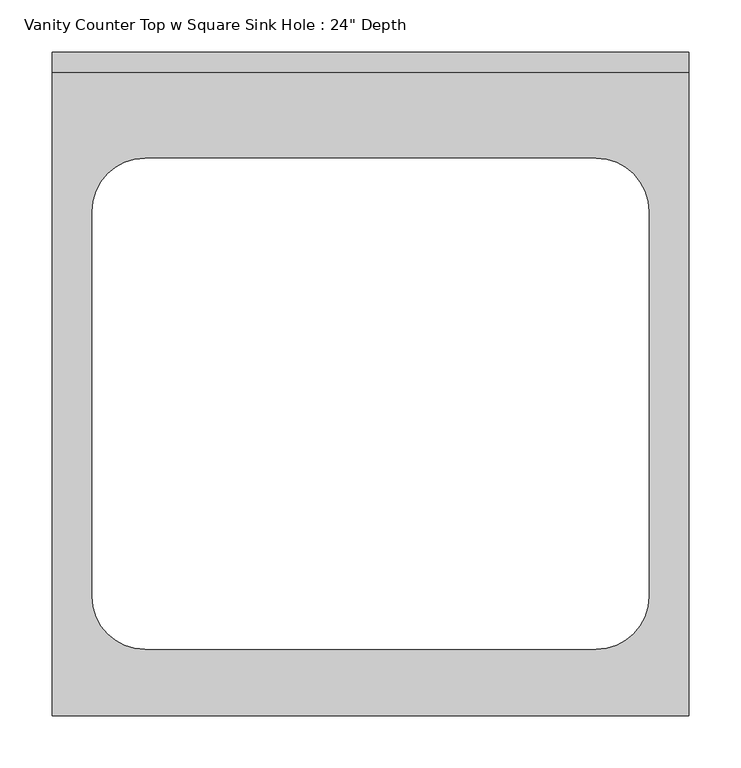
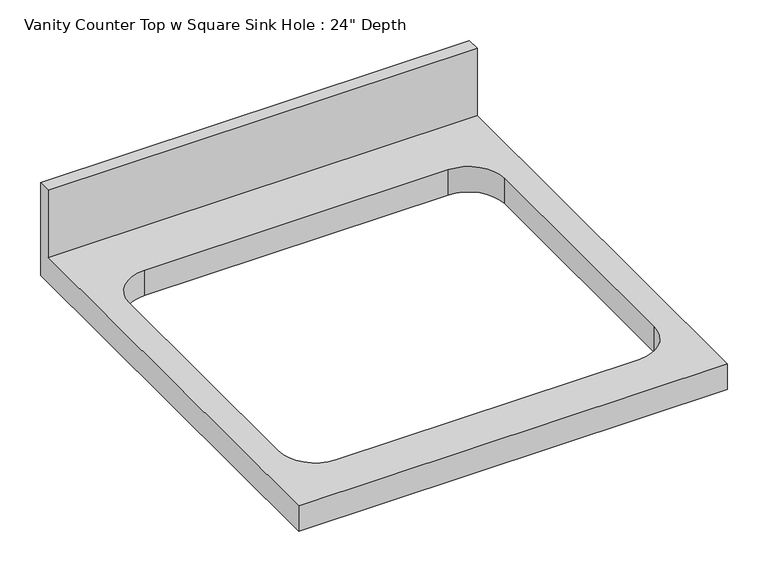
"""IFC4 building model written with IfcOpenShell, lengths in millimetres: furniture geometry."""

from ifc_helpers import new_model, si_unit, frame, origin, place, context, project, spatial, polyline, circle_curve, source, transform, mapped, element, save
from ifc_brep_helpers import plane_surface, revolved_surface, advanced_brep


def furniture_9bca86e0(model_context):
    return source(origin(), model_context, "Body", "AdvancedBrep", [
        advanced_brep(
        [(-1268.7247951, -635.0, 787.4), (-659.1247951, -635.0, 787.4), (-659.1247951, -19.05, 787.4), (-1268.7247951, -19.05, 787.4), (-1230.6247951, -152.4, 787.4), (-1179.8247951, -101.6, 787.4), (-748.0247951, -101.6, 787.4), (-697.2247951, -152.4, 787.4), (-697.2247951, -520.7, 787.4), (-748.0247951, -571.5, 787.4), (-1179.8247951, -571.5, 787.4), (-1230.6247951, -520.7, 787.4), (-659.1247951, 0.0, 749.3), (-659.1247951, -635.0, 749.3), (-1268.7247951, -635.0, 749.3), (-1268.7247951, 0.0, 749.3), (-1179.8247951, -101.6, 749.3), (-1230.6247951, -152.4, 749.3), (-1230.6247951, -520.7, 749.3), (-1179.8247951, -571.5, 749.3), (-748.0247951, -571.5, 749.3), (-697.2247951, -520.7, 749.3), (-697.2247951, -152.4, 749.3), (-748.0247951, -101.6, 749.3), (-1268.7247951, 0.0, 889.0), (-659.1247951, 0.0, 889.0), (-1268.7247951, -19.05, 889.0), (-659.1247951, -19.05, 889.0)],
        [
            (0, 1),
            (1, 2),
            (2, 3),
            (3, 0),
            (4, 5, circle_curve(frame((-1179.8247951, -152.4, 787.4), z_axis=(0.0, 0.0, -1.0), x_axis=(1.0, 0.0, 0.0)), 50.8)),
            (5, 6),
            (6, 7, circle_curve(frame((-748.0247951, -152.4, 787.4), z_axis=(0.0, 0.0, -1.0), x_axis=(1.0, 0.0, 0.0)), 50.8)),
            (7, 8),
            (8, 9, circle_curve(frame((-748.0247951, -520.7, 787.4), z_axis=(0.0, 0.0, -1.0), x_axis=(1.0, 0.0, 0.0)), 50.8)),
            (9, 10),
            (10, 11, circle_curve(frame((-1179.8247951, -520.7, 787.4), z_axis=(0.0, 0.0, -1.0), x_axis=(1.0, 0.0, 0.0)), 50.8)),
            (11, 4),
            (12, 13),
            (13, 14),
            (14, 15),
            (15, 12),
            (16, 17, circle_curve(frame((-1179.8247951, -152.4, 749.3), z_axis=(0.0, 0.0, 1.0), x_axis=(1.0, 0.0, 0.0)), 50.8)),
            (17, 18),
            (18, 19, circle_curve(frame((-1179.8247951, -520.7, 749.3), z_axis=(0.0, 0.0, 1.0), x_axis=(1.0, 0.0, 0.0)), 50.8)),
            (19, 20),
            (20, 21, circle_curve(frame((-748.0247951, -520.7, 749.3), z_axis=(0.0, 0.0, 1.0), x_axis=(1.0, 0.0, 0.0)), 50.8)),
            (21, 22),
            (22, 23, circle_curve(frame((-748.0247951, -152.4, 749.3), z_axis=(0.0, 0.0, 1.0), x_axis=(1.0, 0.0, 0.0)), 50.8)),
            (23, 16),
            (15, 24),
            (24, 25),
            (25, 12),
            (14, 0),
            (3, 26),
            (26, 24),
            (13, 1),
            (25, 27),
            (27, 2),
            (26, 27),
            (4, 17),
            (16, 5),
            (11, 18),
            (10, 19),
            (9, 20),
            (8, 21),
            (7, 22),
            (6, 23),
        ],
        [
            plane_surface(frame((-1268.7247951, 0.0, 787.4), z_axis=(0.0, 0.0, 1.0), x_axis=(-1.0, 0.0, 0.0))),
            plane_surface(frame((-1268.7247951, 0.0, 749.3), z_axis=(0.0, 0.0, -1.0), x_axis=(1.0, 0.0, 0.0))),
            plane_surface(frame((-659.1247951, 0.0, 787.4), z_axis=(0.0, 1.0, 0.0), x_axis=(0.0, 0.0, -1.0))),
            plane_surface(frame((-1268.7247951, 0.0, 787.4), z_axis=(-1.0, 0.0, 0.0), x_axis=(0.0, 0.0, -1.0))),
            plane_surface(frame((-1268.7247951, -635.0, 787.4), z_axis=(0.0, -1.0, 0.0), x_axis=(0.0, 0.0, -1.0))),
            plane_surface(frame((-659.1247951, -635.0, 787.4), z_axis=(1.0, 0.0, 0.0), x_axis=(0.0, 0.0, -1.0))),
            plane_surface(frame((-1268.7247951, 0.0, 889.0), z_axis=(0.0, 0.0, 1.0), x_axis=(0.0, -1.0, 0.0))),
            plane_surface(frame((-1268.7247951, -19.05, 889.0), z_axis=(0.0, -1.0, 0.0), x_axis=(0.0, 0.0, -1.0))),
            revolved_surface(polyline([(-1129.0247951000001, -152.4, 787.4), (-1129.0247951000001, -152.4, 749.3)]), (-1179.8247951, -152.4, 749.3), (0.0, 0.0, 1.0)),
            plane_surface(frame((-1230.6247951, -152.4, 787.4), z_axis=(1.0, 0.0, 0.0), x_axis=(0.0, 0.0, -1.0))),
            revolved_surface(polyline([(-1129.0247951000001, -520.7, 787.4), (-1129.0247951000001, -520.7, 749.3)]), (-1179.8247951, -520.7, 749.3), (0.0, 0.0, 1.0)),
            plane_surface(frame((-1179.8247951, -571.5, 787.4), z_axis=(0.0, 1.0, 0.0), x_axis=(0.0, 0.0, -1.0))),
            revolved_surface(polyline([(-697.2247951, -520.7, 787.4), (-697.2247951, -520.7, 749.3)]), (-748.0247951, -520.7, 749.3), (0.0, 0.0, 1.0)),
            plane_surface(frame((-697.2247951, -520.7, 787.4), z_axis=(-1.0, 0.0, 0.0), x_axis=(0.0, 0.0, -1.0))),
            revolved_surface(polyline([(-697.2247951, -152.4, 787.4), (-697.2247951, -152.4, 749.3)]), (-748.0247951, -152.4, 749.3), (0.0, 0.0, 1.0)),
            plane_surface(frame((-748.0247951, -101.6, 787.4), z_axis=(0.0, -1.0, 0.0), x_axis=(0.0, 0.0, -1.0))),
        ],
        [
            (0, [[1, 2, 3, 4], [5, 6, 7, 8, 9, 10, 11, 12]]),
            (1, [[13, 14, 15, 16], [17, 18, 19, 20, 21, 22, 23, 24]]),
            (2, [[-16, 25, 26, 27]]),
            (3, [[-15, 28, -4, 29, 30, -25]]),
            (4, [[-1, -28, -14, 31]]),
            (5, [[-13, -27, 32, 33, -2, -31]]),
            (6, [[-30, 34, -32, -26]]),
            (7, [[-34, -29, -3, -33]]),
            (8, [[35, -17, 36, -5]]),
            (9, [[-35, -12, 37, -18]]),
            (10, [[-37, -11, 38, -19]]),
            (11, [[-38, -10, 39, -20]]),
            (12, [[-39, -9, 40, -21]]),
            (13, [[-40, -8, 41, -22]]),
            (14, [[-41, -7, 42, -23]]),
            (15, [[-36, -24, -42, -6]]),
        ],
    ),
    ])


if __name__ == "__main__":
    model = new_model("IFC4")
    model_context = context("Model", 3, world=origin())
    ifc_project = project(units=[si_unit("LENGTHUNIT", "METRE", prefix="MILLI")], contexts=[model_context])
    site = spatial("IfcSite", under=ifc_project)
    building = spatial("IfcBuilding", under=site)
    placement = place(None, origin())
    furniture_shape = furniture_9bca86e0(model_context)
    element("IfcFurniture", 1, ObjectType="Vanity Counter Top w Square Sink Hole : 24\" Depth", at=placement, inside=building, context=model_context, shape_type="MappedRepresentation", body=[
        mapped(furniture_shape, transform((0.0, 0.0, 0.0), x_axis=(1.0, 0.0, 0.0), y_axis=(0.0, 1.0, 0.0), z_axis=(0.0, 0.0, 1.0))),
    ])
    save(model, "model.ifc")

# Revit data of these elements
# Type "Vanity Counter Top w Square Sink Hole : 24\" Depth"
#   Assembly Code = "C1030400"
#   Counter Thickness = 0' - 1 1/2"
#   Depth = 2' - 1"
#   Height = 2' - 7"
#   Length [instance default] = 4' - 0"
#   Sink Location [instance default] = 2' - 0"
#   Sink Location To Wall [instance default] = 0' - 4 1/2"
#   Sink Opening Depth [instance default] = 1' - 5 1/2"
#   Sink Opening Width [instance default] = 1' - 8"
#   Counter Top Material = none
# Element 1 (IfcFurniture, "Vanity Counter Top w Square Sink Hole : 24\" Depth")
#   Length = 2' - 0"
#   Sink Location = 1' - 0"
#   Materials on its faces: "Counter Top"
# Materials
#   "Counter Top": class "Wood", colour RGB 226 177 128, transparency 0
